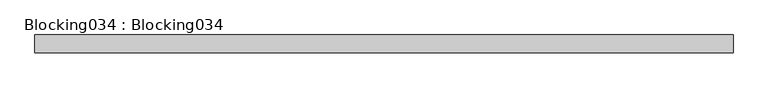
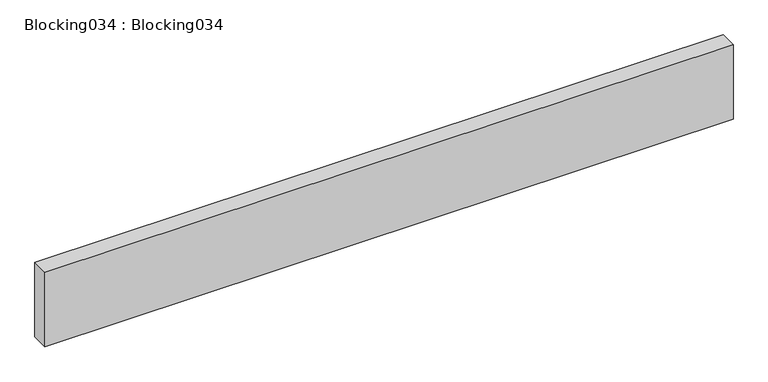
"""IFC4 building model written with IfcOpenShell, lengths in millimetres: proxy geometry, Blocking034 : Blocking034."""

from ifc_helpers import new_model, si_unit, frame, origin, place, context, project, spatial, polyline, outline, extrude, source, transform, mapped, element, save


def blocking034_blocking034_6565a4e6(model_context):
    return source(origin(), model_context, "Body", "SweptSolid", [
        extrude(outline(polyline([(3694.2883192, 9646.2484232), (3694.2883192, 9697.0484232), (5694.2883192, 9697.0484232), (5694.2883192, 9646.2484232), (3694.2883192, 9646.2484232)])), frame((0.0, 0.0, 39528.496), z_axis=(0.0, 0.0, 1.0), x_axis=(1.0, 0.0, 0.0)), (0.0, 0.0, 1.0), 228.6),
    ])


if __name__ == "__main__":
    model = new_model("IFC4")
    model_context = context("Model", 3, world=origin())
    ifc_project = project(units=[si_unit("LENGTHUNIT", "METRE", prefix="MILLI")], contexts=[model_context])
    site = spatial("IfcSite", under=ifc_project)
    building = spatial("IfcBuilding", under=site)
    placement = place(None, origin())
    blocking034_blocking034_shape = blocking034_blocking034_6565a4e6(model_context)
    element("IfcBuildingElementProxy", 1, Name="Blocking034 : Blocking034", ObjectType="Blocking034 : Blocking034", at=placement, inside=building, context=model_context, shape_type="MappedRepresentation", body=[
        mapped(blocking034_blocking034_shape, transform((0.0, 0.0, 0.0), x_axis=(1.0, 0.0, 0.0), y_axis=(0.0, 1.0, 0.0), z_axis=(0.0, 0.0, 1.0))),
    ])
    save(model, "model.ifc")

# Revit data of these elements
# Type "Blocking034 : Blocking034"
#   NameOverride = "Blocking034"
# Element 1 (IfcBuildingElementProxy, "Blocking034 : Blocking034")
#   Materials on its faces: "WOOD BLOCKING AS REQUIRED"
# Materials
#   "WOOD BLOCKING AS REQUIRED": class "Unassigned", colour RGB 166 124 85, transparency 0, Cost = 0
